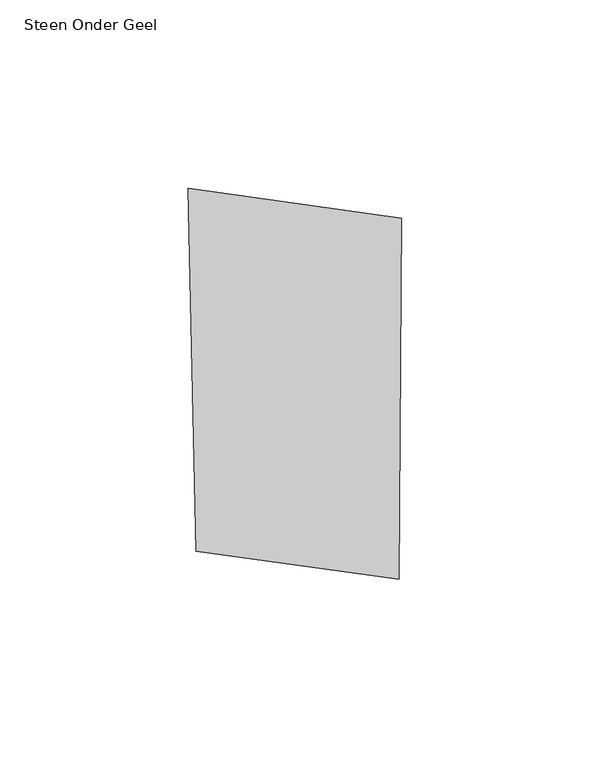
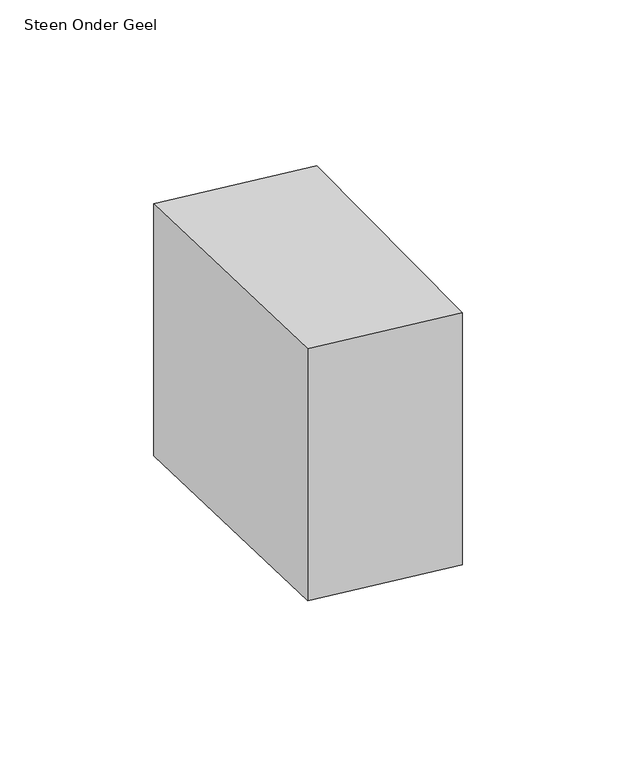
"""IFC4 building model written with IfcOpenShell, lengths in millimetres: proxy geometry, 00_GMA_steen_versie_4 : Steen Onder Geel."""

import ifcopenshell
import ifcopenshell.guid

model = None  # the IFC model being written
_history = None  # IfcOwnerHistory: only IFC2X3 demands one
_inside = {}  # id of a spatial element -> (the spatial element, [elements in it])
_under = {}  # id of a project, library or spatial element -> (it, [spatial elements below it])
_declared = {}  # id of a project -> (the project, [libraries it declares])
_typed = {}  # id of a type object -> (the type object, [elements of that type])
_made_of = {}  # id of a material, layer set ... -> (it, [elements and type objects made of it])


def new_model(schema):
    """Start an empty IFC model of exactly this schema.

    Asked for "IFC4X3", IfcOpenShell would pick the latest addendum, in which some entities
    have other attributes; the version numbers below select the first issue.
    IFC2X3 requires an IfcOwnerHistory on every rooted entity: one is made here for all.
    """
    global model, _history
    if schema == "IFC4X3":
        model = ifcopenshell.file(schema_version=(4, 3, 0, 0))
    else:
        model = ifcopenshell.file(schema=schema)
    _inside.clear()
    _under.clear()
    _declared.clear()
    _typed.clear()
    _made_of.clear()
    _history = None
    if model.schema == "IFC2X3":
        org = make("IfcOrganization", Name="unknown")
        user = make(
            "IfcPersonAndOrganization",
            ThePerson=make("IfcPerson", FamilyName="unknown"),
            TheOrganization=org,
        )
        app = make(
            "IfcApplication",
            ApplicationDeveloper=org,
            Version="unknown",
            ApplicationFullName="unknown",
            ApplicationIdentifier="unknown",
        )
        _history = make(
            "IfcOwnerHistory",
            OwningUser=user,
            OwningApplication=app,
            ChangeAction="ADDED",
            CreationDate=0,
        )
    return model


def make(cls, **values):
    """One entity of the class cls with the attributes given. An attribute that is None is left unset."""
    return model.create_entity(
        cls, **{name: value for name, value in values.items() if value is not None}
    )


def rooted(cls, **values):
    """An entity with a GlobalId (a new one), such as an element, a storey or a relation."""
    return make(cls, GlobalId=ifcopenshell.guid.new(), OwnerHistory=_history, **values)


def si_unit(unit_type, name, prefix=None):
    """IfcSIUnit, for example si_unit("LENGTHUNIT", "METRE", prefix="MILLI")."""
    return make("IfcSIUnit", UnitType=unit_type, Prefix=prefix, Name=name)


def assignment(units):
    """IfcUnitAssignment: the units of a project."""
    return None if units is None else make("IfcUnitAssignment", Units=units)


def point(xyz):
    """IfcCartesianPoint."""
    return None if xyz is None else make("IfcCartesianPoint", Coordinates=xyz)


def direction(xyz):
    """IfcDirection."""
    return None if xyz is None else make("IfcDirection", DirectionRatios=xyz)


def frame(location, z_axis=None, x_axis=None):
    """IfcAxis2Placement3D, a coordinate frame: its origin and axes. An axis left out is left unset."""
    return make(
        "IfcAxis2Placement3D",
        Location=point(location),
        Axis=direction(z_axis),
        RefDirection=direction(x_axis),
    )


def origin():
    """The frame at (0, 0, 0) with its axes left unset."""
    return frame((0.0, 0.0, 0.0))


def origin_with_axes():
    """The frame at (0, 0, 0) with the z axis (0, 0, 1) and the x axis (1, 0, 0) written out."""
    return frame((0.0, 0.0, 0.0), z_axis=(0.0, 0.0, 1.0), x_axis=(1.0, 0.0, 0.0))


def place(relative_to, where):
    """IfcLocalPlacement: puts the frame where relative to a parent placement (None: the world)."""
    return make(
        "IfcLocalPlacement", PlacementRelTo=relative_to, RelativePlacement=where
    )


def context(
    kind, dimensions, precision=None, world=None, true_north=None, identifier=None
):
    """IfcGeometricRepresentationContext, for example the 3D "Model" context."""
    return make(
        "IfcGeometricRepresentationContext",
        ContextIdentifier=identifier,
        ContextType=kind,
        CoordinateSpaceDimension=dimensions,
        Precision=precision,
        WorldCoordinateSystem=world,
        TrueNorth=true_north,
    )


def project(units=None, contexts=None):
    """IfcProject with its units and contexts."""
    return rooted(
        "IfcProject",
        Name="project",
        RepresentationContexts=contexts,
        UnitsInContext=assignment(units),
    )


def spatial(cls, under=None, at=None, **own):
    """A site, building, storey or space (cls), placed at a placement, below another one or the project."""
    s = rooted(cls, ObjectPlacement=at, **own)
    if under is not None:
        _under.setdefault(under.id(), (under, []))[1].append(s)
    return s


def polyline(points):
    """IfcPolyline through the points."""
    return make("IfcPolyline", Points=[point(p) for p in points])


def outline(outer, holes=None, kind="AREA"):
    """IfcArbitraryClosedProfileDef: a profile drawn as a closed curve; with holes, ...WithVoids."""
    if holes is None:
        return make("IfcArbitraryClosedProfileDef", ProfileType=kind, OuterCurve=outer)
    return make(
        "IfcArbitraryProfileDefWithVoids",
        ProfileType=kind,
        OuterCurve=outer,
        InnerCurves=holes,
    )


def extrude(swept, where, along, depth):
    """IfcExtrudedAreaSolid: the profile swept, set in the frame where, extruded along a direction by depth."""
    return make(
        "IfcExtrudedAreaSolid",
        SweptArea=swept,
        Position=where,
        ExtrudedDirection=direction(along),
        Depth=depth,
    )


def shape(context_of_items, identifier, shape_type, items):
    """IfcShapeRepresentation: the items that make up one representation, for example the "Body"."""
    return make(
        "IfcShapeRepresentation",
        ContextOfItems=context_of_items,
        RepresentationIdentifier=identifier,
        RepresentationType=shape_type,
        Items=items,
    )


def source(mapping_origin, context_of_items, identifier, shape_type, items):
    """IfcRepresentationMap: a shape defined once, which mapped items show again and again."""
    return make(
        "IfcRepresentationMap",
        MappingOrigin=mapping_origin,
        MappedRepresentation=shape(context_of_items, identifier, shape_type, items),
    )


def transform(
    local_origin,
    x_axis=None,
    y_axis=None,
    z_axis=None,
    scale=None,
    scale2=None,
    scale3=None,
    uniform=True,
):
    """IfcCartesianTransformationOperator3D, or its non-uniform kind. x_axis, y_axis, z_axis: its Axis1, 2, 3."""
    if uniform:
        return make(
            "IfcCartesianTransformationOperator3D",
            Axis1=direction(x_axis),
            Axis2=direction(y_axis),
            LocalOrigin=point(local_origin),
            Scale=scale,
            Axis3=direction(z_axis),
        )
    return make(
        "IfcCartesianTransformationOperator3DnonUniform",
        Axis1=direction(x_axis),
        Axis2=direction(y_axis),
        LocalOrigin=point(local_origin),
        Scale=scale,
        Axis3=direction(z_axis),
        Scale2=scale2,
        Scale3=scale3,
    )


def mapped(mapping_source, mapping_target):
    """IfcMappedItem: shows the shape of a source again, moved by a transform."""
    return make(
        "IfcMappedItem", MappingSource=mapping_source, MappingTarget=mapping_target
    )


def made_of(thing, what):
    """Note that an element or type object is made of a material, layer set ...; save() writes the relation."""
    if what is not None:
        _made_of.setdefault(what.id(), (what, []))[1].append(thing)
    return thing


def element(
    cls,
    number,
    at=None,
    inside=None,
    cuts=None,
    type_object=None,
    material=None,
    context=None,
    identifier="Body",
    shape_type=None,
    held_by="IfcProductDefinitionShape",
    body=None,
    shapes=None,
    **own,
):
    """One element of the class cls, such as IfcWall. Its Tag is "e" and its number.

    at: its placement. inside: the storey or other place that contains it. cuts: it is an
    opening in that element (IfcRelVoidsElement). A single representation is given by context,
    identifier, shape_type and body (its items); several are given by shapes. held_by: the class
    of the entity that holds the representations. save() writes the other relations.
    """
    e = rooted(cls, Tag="e%d" % number, ObjectPlacement=at, **own)
    if body is not None:
        shapes = [shape(context, identifier, shape_type, body)]
    if shapes is not None:
        e.Representation = make(held_by, Representations=shapes)
    if inside is not None:
        _inside.setdefault(inside.id(), (inside, []))[1].append(e)
    if cuts is not None:
        rooted(
            "IfcRelVoidsElement", RelatingBuildingElement=cuts, RelatedOpeningElement=e
        )
    if type_object is not None:
        _typed.setdefault(type_object.id(), (type_object, []))[1].append(e)
    return made_of(e, material)


def aggregate(whole, parts):
    """IfcRelAggregates: a whole, such as a stair, and the parts it consists of."""
    return rooted("IfcRelAggregates", RelatingObject=whole, RelatedObjects=parts)


def save(model, path):
    """Write the relations noted so far, then the file.

    IfcRelAggregates (storeys below a building ...), IfcRelContainedInSpatialStructure (elements
    in a storey), IfcRelDefinesByType, IfcRelAssociatesMaterial and IfcRelDeclares: one each for
    every whole, place, type object, material and project.
    """
    for whole, parts in _under.values():
        aggregate(whole, parts)
    for where, things in _inside.values():
        rooted(
            "IfcRelContainedInSpatialStructure",
            RelatedElements=things,
            RelatingStructure=where,
        )
    for kind, things in _typed.values():
        rooted("IfcRelDefinesByType", RelatedObjects=things, RelatingType=kind)
    for what, things in _made_of.values():
        rooted("IfcRelAssociatesMaterial", RelatedObjects=things, RelatingMaterial=what)
    for by, libraries in _declared.values():
        rooted("IfcRelDeclares", RelatingContext=by, RelatedDefinitions=libraries)
    model.write(path)


def steen_onder_geel_30d665b3(model_context):
    return source(origin(), model_context, "Body", "SweptSolid", [
        extrude(outline(polyline([(100.9042723, 114.7127203), (100.2631156, 18.8519275), (46.4677975, 26.294319), (44.3561114, 122.5537298), (100.9042723, 114.7127203)])), origin_with_axes(), (0.0, 0.0, 1.0), 100.0),
    ])


if __name__ == "__main__":
    model = new_model("IFC4")
    model_context = context("Model", 3, world=origin())
    ifc_project = project(units=[si_unit("LENGTHUNIT", "METRE", prefix="MILLI")], contexts=[model_context])
    site = spatial("IfcSite", under=ifc_project)
    building = spatial("IfcBuilding", under=site)
    placement = place(None, origin())
    steen_onder_geel_shape = steen_onder_geel_30d665b3(model_context)
    element("IfcBuildingElementProxy", 1, Name="00_GMA_steen_versie_4 : Steen Onder Geel", ObjectType="00_GMA_steen_versie_4 : Steen Onder Geel", at=placement, inside=building, context=model_context, shape_type="MappedRepresentation", body=[
        mapped(steen_onder_geel_shape, transform((0.0, 0.0, 0.0), x_axis=(1.0, 0.0, 0.0), y_axis=(0.0, 1.0, 0.0), z_axis=(0.0, 0.0, 1.0))),
    ])
    save(model, "model.ifc")

# Revit data of these elements
# Type "00_GMA_steen_versie_4 : Steen Onder Geel"
#   StootVoegHalfBoven [instance default] = 5 mm
#   StootVoegHalf [instance default] = 5 mm
#   StootVoegBreedteOnder = 10 mm
#   StootVoegBreedteBoven = 10 mm
#   Steendikte = 100 mm
#   LintVoegOnderHalf = 0 mm
#   LintVoegOnder = 0 mm
#   LintVoegBovenHalf = 5 mm
#   LintVoegBoven = 10 mm
#   materiaal = 21_steen_geel
#   MateriaalVoeg = none
#   Default Elevation = 0
# Element 1 (IfcBuildingElementProxy, "00_GMA_steen_versie_4 : Steen Onder Geel")
#   Materials on its faces: "21_steen_geel"
# Materials
#   "21_steen_geel": class "Unassigned", colour RGB 202 202 0, transparency 0, Cost = 0
